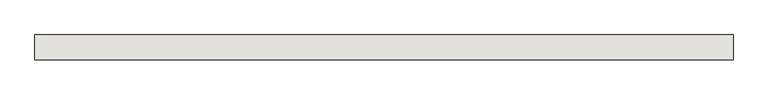
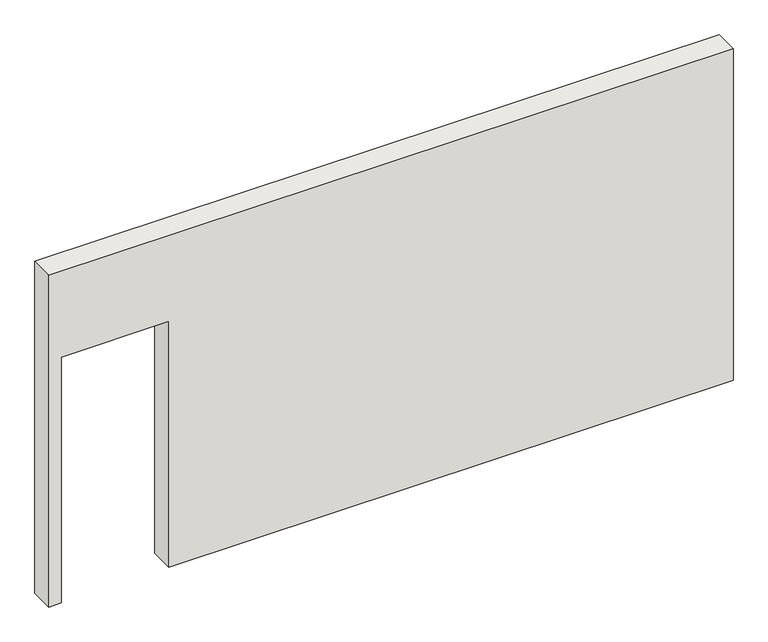
"""IFC4 building model written with IfcOpenShell, lengths in millimetres: wall geometry, Holzwand."""

from ifc_helpers import new_model, si_unit, frame, origin, place, context, project, spatial, polyline, outline, extrude, source, transform, mapped, element, save


def wall_ff0262cd(model_context):
    return source(origin(), model_context, "Body", "SweptSolid", [
        extrude(outline(polyline([(2135.0, 985.7388884), (0.0, 985.7388884), (0.0, 5620.0), (2880.0, 5620.0), (2880.0, 0.0), (0.0, 0.0), (0.0, 100.7388884), (2135.0, 100.7388884), (2135.0, 985.7388884)])), frame((0.0, 0.0, 0.0), z_axis=(0.0, 1.0, 0.0), x_axis=(0.0, 0.0, 1.0)), (0.0, 0.0, 1.0), 200.0),
    ])


if __name__ == "__main__":
    model = new_model("IFC4")
    model_context = context("Model", 3, world=origin())
    ifc_project = project(units=[si_unit("LENGTHUNIT", "METRE", prefix="MILLI")], contexts=[model_context])
    site = spatial("IfcSite", under=ifc_project)
    building = spatial("IfcBuilding", under=site)
    placement = place(None, origin())
    wall_shape = wall_ff0262cd(model_context)
    element("IfcWall", 1, ObjectType="Holzwand", at=placement, inside=building, context=model_context, shape_type="MappedRepresentation", body=[
        mapped(wall_shape, transform((0.0, 0.0, 0.0), x_axis=(1.0, 0.0, 0.0), y_axis=(0.0, 1.0, 0.0), z_axis=(0.0, 0.0, 1.0))),
    ])
    save(model, "model.ifc")

# Revit data of these elements
# Element 1 (IfcWall, "Holzwand")
#   Materials on its faces: "holzschalung"
# Materials
#   "holzschalung": class "Unassigned", colour RGB 128 128 128, transparency 0
